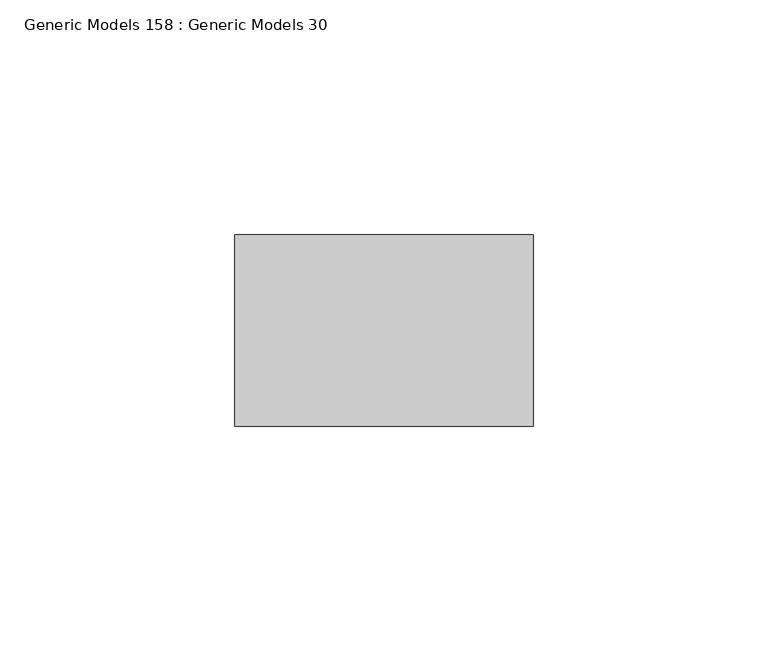
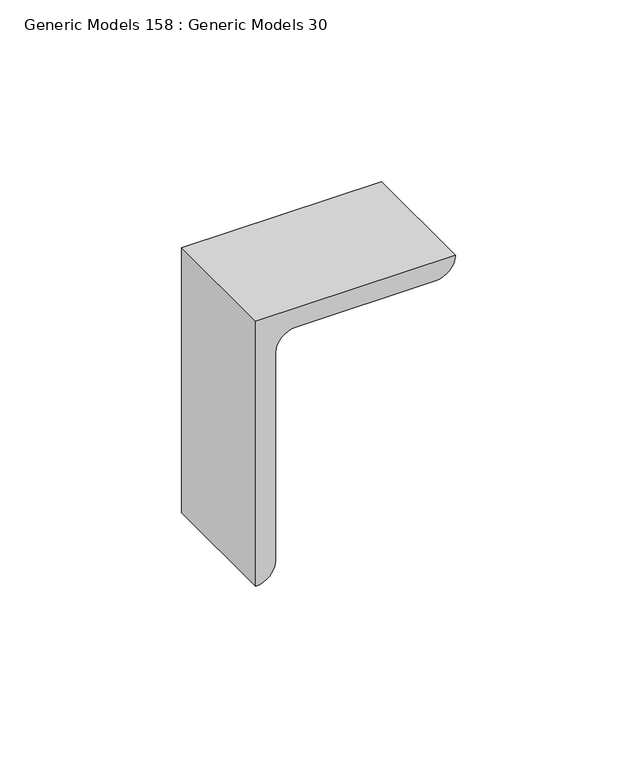
"""IFC4 building model written with IfcOpenShell, lengths in millimetres: proxy geometry, Generic Models 158 : Generic Models 30."""

from ifc_helpers import new_model, si_unit, point, frame, frame_2d, origin, place, context, project, spatial, polyline, circle_curve, trimmed, segment, composite_curve, outline, extrude, source, transform, mapped, element, save


def generic_models_158_generic_models_30_ae75cb85(model_context):
    return source(origin(), model_context, "Body", "SweptSolid", [
        extrude(outline(composite_curve([segment(polyline([(268865.4044757, 34434.4590778), (268776.5044757, 34434.4590778)]), True, "CONTINUOUS"), segment(trimmed(circle_curve(frame_2d((268782.8544757, 34434.4590778)), 6.35), [point((268776.5044757, 34434.4590778))], [point((268782.8544757, 34440.8090778))], False, "CARTESIAN"), True, "CONTINUOUS"), segment(polyline([(268782.8544757, 34440.8090778), (268852.7044757, 34440.8090778)]), True, "CONTINUOUS"), segment(trimmed(circle_curve(frame_2d((268852.7044757, 34447.1590778)), 6.35), [point((268852.7044757, 34440.8090778))], [point((268859.0544757, 34447.1590778))], True, "CARTESIAN"), True, "CONTINUOUS"), segment(polyline([(268859.0544757, 34447.1590778), (268859.0544757, 34491.6090778)]), True, "CONTINUOUS"), segment(trimmed(circle_curve(frame_2d((268865.4044757, 34491.6090778)), 6.35), [point((268859.0544757, 34491.6090778))], [point((268865.4044757, 34497.9590778))], False, "CARTESIAN"), True, "CONTINUOUS"), segment(polyline([(268865.4044757, 34497.9590778), (268865.4044757, 34434.4590778)]), True, "CONTINUOUS")], self_intersect=False)), frame((0.0, 41007.6196612, 0.0), z_axis=(0.0, 1.0, 0.0), x_axis=(0.0, 0.0, 1.0)), (0.0, 0.0, 1.0), 40.7035),
    ])


if __name__ == "__main__":
    model = new_model("IFC4")
    model_context = context("Model", 3, world=origin())
    ifc_project = project(units=[si_unit("LENGTHUNIT", "METRE", prefix="MILLI")], contexts=[model_context])
    site = spatial("IfcSite", under=ifc_project)
    building = spatial("IfcBuilding", under=site)
    placement = place(None, origin())
    generic_models_158_generic_models_30_shape = generic_models_158_generic_models_30_ae75cb85(model_context)
    element("IfcBuildingElementProxy", 1, Name="Generic Models 158 : Generic Models 30", ObjectType="Generic Models 158 : Generic Models 30", at=placement, inside=building, context=model_context, shape_type="MappedRepresentation", body=[
        mapped(generic_models_158_generic_models_30_shape, transform((0.0, 0.0, 0.0), x_axis=(1.0, 0.0, 0.0), y_axis=(0.0, 1.0, 0.0), z_axis=(0.0, 0.0, 1.0))),
    ])
    save(model, "model.ifc")

# Revit data of these elements
# Element 1 (IfcBuildingElementProxy, "Generic Models 158 : Generic Models 30")
#   Materials on its faces: "GALV 3 1/2\"X 2 1/2\" X 1/4\" STEEL ANGLE - WELD TO VERTICAL STEEL ANGLE"
# Materials
#   "GALV 3 1/2\"X 2 1/2\" X 1/4\" STEEL ANGLE - WELD TO VERTICAL STEEL ANGLE": class "Metal", colour RGB 199 199 199, transparency 0, Description = "Structural steel, ASTM A36 Grade B, mill finish", Cost = 0
